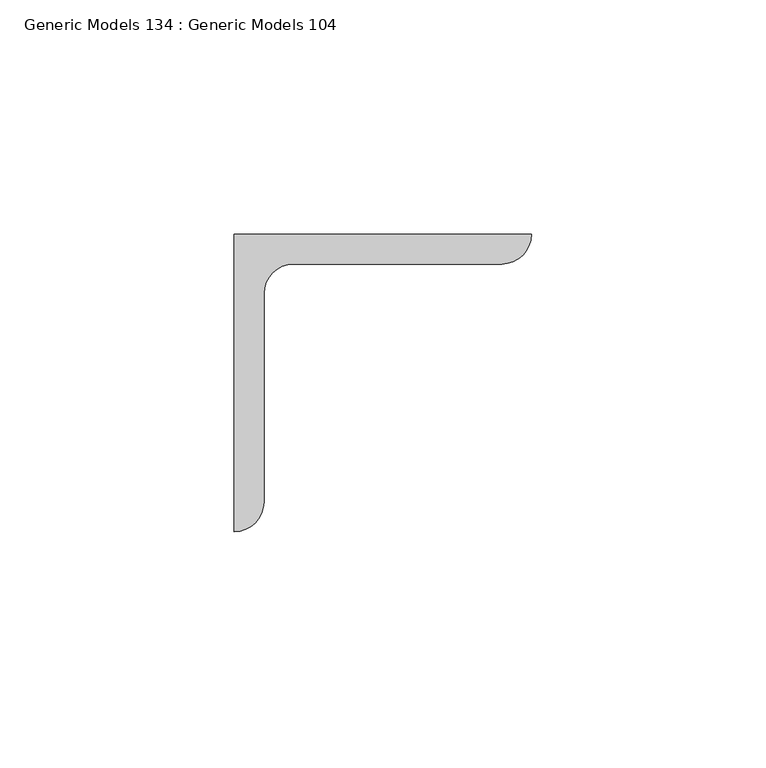
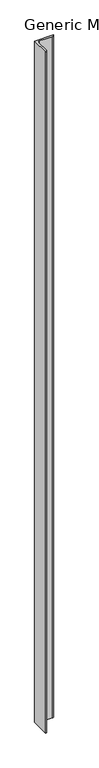
"""IFC4 building model written with IfcOpenShell, lengths in millimetres: proxy geometry, Generic Models 134 : Generic Models 104."""

import ifcopenshell
import ifcopenshell.guid

model = None  # the IFC model being written
_history = None  # IfcOwnerHistory: only IFC2X3 demands one
_inside = {}  # id of a spatial element -> (the spatial element, [elements in it])
_under = {}  # id of a project, library or spatial element -> (it, [spatial elements below it])
_declared = {}  # id of a project -> (the project, [libraries it declares])
_typed = {}  # id of a type object -> (the type object, [elements of that type])
_made_of = {}  # id of a material, layer set ... -> (it, [elements and type objects made of it])


def new_model(schema):
    """Start an empty IFC model of exactly this schema.

    Asked for "IFC4X3", IfcOpenShell would pick the latest addendum, in which some entities
    have other attributes; the version numbers below select the first issue.
    IFC2X3 requires an IfcOwnerHistory on every rooted entity: one is made here for all.
    """
    global model, _history
    if schema == "IFC4X3":
        model = ifcopenshell.file(schema_version=(4, 3, 0, 0))
    else:
        model = ifcopenshell.file(schema=schema)
    _inside.clear()
    _under.clear()
    _declared.clear()
    _typed.clear()
    _made_of.clear()
    _history = None
    if model.schema == "IFC2X3":
        org = make("IfcOrganization", Name="unknown")
        user = make(
            "IfcPersonAndOrganization",
            ThePerson=make("IfcPerson", FamilyName="unknown"),
            TheOrganization=org,
        )
        app = make(
            "IfcApplication",
            ApplicationDeveloper=org,
            Version="unknown",
            ApplicationFullName="unknown",
            ApplicationIdentifier="unknown",
        )
        _history = make(
            "IfcOwnerHistory",
            OwningUser=user,
            OwningApplication=app,
            ChangeAction="ADDED",
            CreationDate=0,
        )
    return model


def make(cls, **values):
    """One entity of the class cls with the attributes given. An attribute that is None is left unset."""
    return model.create_entity(
        cls, **{name: value for name, value in values.items() if value is not None}
    )


def rooted(cls, **values):
    """An entity with a GlobalId (a new one), such as an element, a storey or a relation."""
    return make(cls, GlobalId=ifcopenshell.guid.new(), OwnerHistory=_history, **values)


def si_unit(unit_type, name, prefix=None):
    """IfcSIUnit, for example si_unit("LENGTHUNIT", "METRE", prefix="MILLI")."""
    return make("IfcSIUnit", UnitType=unit_type, Prefix=prefix, Name=name)


def assignment(units):
    """IfcUnitAssignment: the units of a project."""
    return None if units is None else make("IfcUnitAssignment", Units=units)


def point(xyz):
    """IfcCartesianPoint."""
    return None if xyz is None else make("IfcCartesianPoint", Coordinates=xyz)


def direction(xyz):
    """IfcDirection."""
    return None if xyz is None else make("IfcDirection", DirectionRatios=xyz)


def frame(location, z_axis=None, x_axis=None):
    """IfcAxis2Placement3D, a coordinate frame: its origin and axes. An axis left out is left unset."""
    return make(
        "IfcAxis2Placement3D",
        Location=point(location),
        Axis=direction(z_axis),
        RefDirection=direction(x_axis),
    )


def frame_2d(location, x_axis=None):
    """IfcAxis2Placement2D, a coordinate frame in the plane: its origin and x axis."""
    return make(
        "IfcAxis2Placement2D", Location=point(location), RefDirection=direction(x_axis)
    )


def origin():
    """The frame at (0, 0, 0) with its axes left unset."""
    return frame((0.0, 0.0, 0.0))


def place(relative_to, where):
    """IfcLocalPlacement: puts the frame where relative to a parent placement (None: the world)."""
    return make(
        "IfcLocalPlacement", PlacementRelTo=relative_to, RelativePlacement=where
    )


def context(
    kind, dimensions, precision=None, world=None, true_north=None, identifier=None
):
    """IfcGeometricRepresentationContext, for example the 3D "Model" context."""
    return make(
        "IfcGeometricRepresentationContext",
        ContextIdentifier=identifier,
        ContextType=kind,
        CoordinateSpaceDimension=dimensions,
        Precision=precision,
        WorldCoordinateSystem=world,
        TrueNorth=true_north,
    )


def project(units=None, contexts=None):
    """IfcProject with its units and contexts."""
    return rooted(
        "IfcProject",
        Name="project",
        RepresentationContexts=contexts,
        UnitsInContext=assignment(units),
    )


def spatial(cls, under=None, at=None, **own):
    """A site, building, storey or space (cls), placed at a placement, below another one or the project."""
    s = rooted(cls, ObjectPlacement=at, **own)
    if under is not None:
        _under.setdefault(under.id(), (under, []))[1].append(s)
    return s


def polyline(points):
    """IfcPolyline through the points."""
    return make("IfcPolyline", Points=[point(p) for p in points])


def circle_curve(where, radius):
    """IfcCircle in the frame where."""
    return make("IfcCircle", Position=where, Radius=radius)


def trimmed(basis, trim1, trim2, sense, master):
    """IfcTrimmedCurve: the piece of a basis curve between two trims."""
    return make(
        "IfcTrimmedCurve",
        BasisCurve=basis,
        Trim1=trim1,
        Trim2=trim2,
        SenseAgreement=sense,
        MasterRepresentation=master,
    )


def segment(curve, same_sense, transition):
    """IfcCompositeCurveSegment."""
    return make(
        "IfcCompositeCurveSegment",
        Transition=transition,
        SameSense=same_sense,
        ParentCurve=curve,
    )


def composite_curve(segments, self_intersect=None):
    """IfcCompositeCurve: segments joined end to end."""
    return make("IfcCompositeCurve", Segments=segments, SelfIntersect=self_intersect)


def outline(outer, holes=None, kind="AREA"):
    """IfcArbitraryClosedProfileDef: a profile drawn as a closed curve; with holes, ...WithVoids."""
    if holes is None:
        return make("IfcArbitraryClosedProfileDef", ProfileType=kind, OuterCurve=outer)
    return make(
        "IfcArbitraryProfileDefWithVoids",
        ProfileType=kind,
        OuterCurve=outer,
        InnerCurves=holes,
    )


def extrude(swept, where, along, depth):
    """IfcExtrudedAreaSolid: the profile swept, set in the frame where, extruded along a direction by depth."""
    return make(
        "IfcExtrudedAreaSolid",
        SweptArea=swept,
        Position=where,
        ExtrudedDirection=direction(along),
        Depth=depth,
    )


def shape(context_of_items, identifier, shape_type, items):
    """IfcShapeRepresentation: the items that make up one representation, for example the "Body"."""
    return make(
        "IfcShapeRepresentation",
        ContextOfItems=context_of_items,
        RepresentationIdentifier=identifier,
        RepresentationType=shape_type,
        Items=items,
    )


def source(mapping_origin, context_of_items, identifier, shape_type, items):
    """IfcRepresentationMap: a shape defined once, which mapped items show again and again."""
    return make(
        "IfcRepresentationMap",
        MappingOrigin=mapping_origin,
        MappedRepresentation=shape(context_of_items, identifier, shape_type, items),
    )


def transform(
    local_origin,
    x_axis=None,
    y_axis=None,
    z_axis=None,
    scale=None,
    scale2=None,
    scale3=None,
    uniform=True,
):
    """IfcCartesianTransformationOperator3D, or its non-uniform kind. x_axis, y_axis, z_axis: its Axis1, 2, 3."""
    if uniform:
        return make(
            "IfcCartesianTransformationOperator3D",
            Axis1=direction(x_axis),
            Axis2=direction(y_axis),
            LocalOrigin=point(local_origin),
            Scale=scale,
            Axis3=direction(z_axis),
        )
    return make(
        "IfcCartesianTransformationOperator3DnonUniform",
        Axis1=direction(x_axis),
        Axis2=direction(y_axis),
        LocalOrigin=point(local_origin),
        Scale=scale,
        Axis3=direction(z_axis),
        Scale2=scale2,
        Scale3=scale3,
    )


def mapped(mapping_source, mapping_target):
    """IfcMappedItem: shows the shape of a source again, moved by a transform."""
    return make(
        "IfcMappedItem", MappingSource=mapping_source, MappingTarget=mapping_target
    )


def made_of(thing, what):
    """Note that an element or type object is made of a material, layer set ...; save() writes the relation."""
    if what is not None:
        _made_of.setdefault(what.id(), (what, []))[1].append(thing)
    return thing


def element(
    cls,
    number,
    at=None,
    inside=None,
    cuts=None,
    type_object=None,
    material=None,
    context=None,
    identifier="Body",
    shape_type=None,
    held_by="IfcProductDefinitionShape",
    body=None,
    shapes=None,
    **own,
):
    """One element of the class cls, such as IfcWall. Its Tag is "e" and its number.

    at: its placement. inside: the storey or other place that contains it. cuts: it is an
    opening in that element (IfcRelVoidsElement). A single representation is given by context,
    identifier, shape_type and body (its items); several are given by shapes. held_by: the class
    of the entity that holds the representations. save() writes the other relations.
    """
    e = rooted(cls, Tag="e%d" % number, ObjectPlacement=at, **own)
    if body is not None:
        shapes = [shape(context, identifier, shape_type, body)]
    if shapes is not None:
        e.Representation = make(held_by, Representations=shapes)
    if inside is not None:
        _inside.setdefault(inside.id(), (inside, []))[1].append(e)
    if cuts is not None:
        rooted(
            "IfcRelVoidsElement", RelatingBuildingElement=cuts, RelatedOpeningElement=e
        )
    if type_object is not None:
        _typed.setdefault(type_object.id(), (type_object, []))[1].append(e)
    return made_of(e, material)


def aggregate(whole, parts):
    """IfcRelAggregates: a whole, such as a stair, and the parts it consists of."""
    return rooted("IfcRelAggregates", RelatingObject=whole, RelatedObjects=parts)


def save(model, path):
    """Write the relations noted so far, then the file.

    IfcRelAggregates (storeys below a building ...), IfcRelContainedInSpatialStructure (elements
    in a storey), IfcRelDefinesByType, IfcRelAssociatesMaterial and IfcRelDeclares: one each for
    every whole, place, type object, material and project.
    """
    for whole, parts in _under.values():
        aggregate(whole, parts)
    for where, things in _inside.values():
        rooted(
            "IfcRelContainedInSpatialStructure",
            RelatedElements=things,
            RelatingStructure=where,
        )
    for kind, things in _typed.values():
        rooted("IfcRelDefinesByType", RelatedObjects=things, RelatingType=kind)
    for what, things in _made_of.values():
        rooted("IfcRelAssociatesMaterial", RelatedObjects=things, RelatingMaterial=what)
    for by, libraries in _declared.values():
        rooted("IfcRelDeclares", RelatingContext=by, RelatedDefinitions=libraries)
    model.write(path)


def generic_models_134_generic_models_104_a682e9e6(model_context):
    return source(origin(), model_context, "Body", "SweptSolid", [
        extrude(outline(composite_curve([segment(polyline([(33383.5340778, 41071.1196612), (33447.0340778, 41071.1196612)]), True, "CONTINUOUS"), segment(trimmed(circle_curve(frame_2d((33440.6840778, 41071.1196612)), 6.35), [point((33447.0340778, 41071.1196612))], [point((33440.6840778, 41064.7696612))], False, "CARTESIAN"), True, "CONTINUOUS"), segment(polyline([(33440.6840778, 41064.7696612), (33396.2340778, 41064.7696612)]), True, "CONTINUOUS"), segment(trimmed(circle_curve(frame_2d((33396.2340778, 41058.4196612)), 6.35), [point((33396.2340778, 41064.7696612))], [point((33389.8840778, 41058.4196612))], True, "CARTESIAN"), True, "CONTINUOUS"), segment(polyline([(33389.8840778, 41058.4196612), (33389.8840778, 41013.9696612)]), True, "CONTINUOUS"), segment(trimmed(circle_curve(frame_2d((33383.5340778, 41013.9696612)), 6.35), [point((33389.8840778, 41013.9696612))], [point((33383.5340778, 41007.6196612))], False, "CARTESIAN"), True, "CONTINUOUS"), segment(polyline([(33383.5340778, 41007.6196612), (33383.5340778, 41071.1196612)]), True, "CONTINUOUS")], self_intersect=False)), frame((0.0, 0.0, 266407.9), z_axis=(0.0, 0.0, 1.0), x_axis=(1.0, 0.0, 0.0)), (0.0, 0.0, 1.0), 2432.1044757),
    ])


if __name__ == "__main__":
    model = new_model("IFC4")
    model_context = context("Model", 3, world=origin())
    ifc_project = project(units=[si_unit("LENGTHUNIT", "METRE", prefix="MILLI")], contexts=[model_context])
    site = spatial("IfcSite", under=ifc_project)
    building = spatial("IfcBuilding", under=site)
    placement = place(None, origin())
    generic_models_134_generic_models_104_shape = generic_models_134_generic_models_104_a682e9e6(model_context)
    element("IfcBuildingElementProxy", 1, Name="Generic Models 134 : Generic Models 104", ObjectType="Generic Models 134 : Generic Models 104", at=placement, inside=building, context=model_context, shape_type="MappedRepresentation", body=[
        mapped(generic_models_134_generic_models_104_shape, transform((0.0, 0.0, 0.0), x_axis=(1.0, 0.0, 0.0), y_axis=(0.0, 1.0, 0.0), z_axis=(0.0, 0.0, 1.0))),
    ])
    save(model, "model.ifc")

# Revit data of these elements
# Element 1 (IfcBuildingElementProxy, "Generic Models 134 : Generic Models 104")
#   Materials on its faces: "(2) BACK/BACK GALVANIZED ANGLES (2) L2 1/2 X 2 1/2 X 1/4\")"
# Materials
#   "(2) BACK/BACK GALVANIZED ANGLES (2) L2 1/2 X 2 1/2 X 1/4\")": class "Unassigned", colour RGB 211 211 211, transparency 0, Cost = 0
